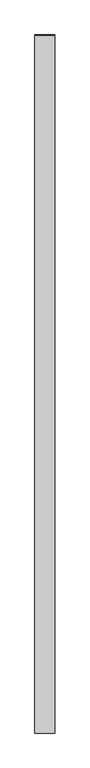
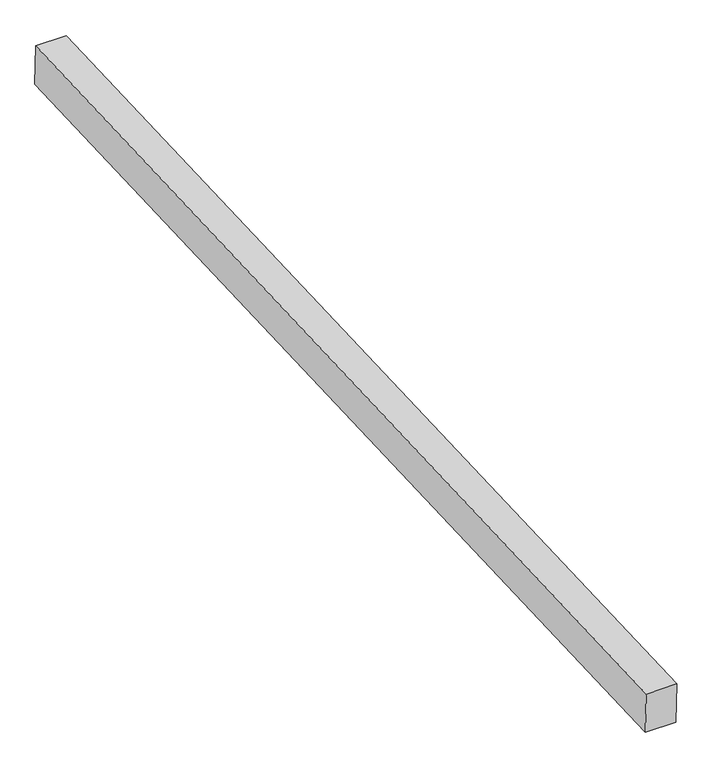
"""IFC4 building model written with IfcOpenShell, lengths in millimetres: proxy geometry, Generic Models 7:Generic Models 1:8:Generic Models 1:8 : Generic Models 7:Generic Models 1:337419:6 : Generic Models 7:Generic Models 1:8:Generic Models 1:8 : Generic Models 7:Generic Models 1:337419:315935."""

from ifc_helpers import new_model, si_unit, frame, origin, place, context, project, spatial, polyline, outline, extrude, source, transform, mapped, element, save


def generic_models_e63649a8(model_context):
    return source(origin(), model_context, "Body", "SweptSolid", [
        extrude(outline(polyline([(-580626.555738, 3844.0209448), (-575753.6328438, 4047.0593987), (-575746.0659221, 3856.7093942), (-580618.6251193, 3653.6860944), (-580626.555738, 3844.0209448)])), frame((593665.061724, 0.0, 0.0), z_axis=(1.0, 0.0, 0.0), x_axis=(0.0, 1.0, 0.0)), (0.0, 0.0, 1.0), 139.7),
    ])


if __name__ == "__main__":
    model = new_model("IFC4")
    model_context = context("Model", 3, world=origin())
    ifc_project = project(units=[si_unit("LENGTHUNIT", "METRE", prefix="MILLI")], contexts=[model_context])
    site = spatial("IfcSite", under=ifc_project)
    building = spatial("IfcBuilding", under=site)
    placement = place(None, origin())
    generic_models_shape = generic_models_e63649a8(model_context)
    element("IfcBuildingElementProxy", 1, Name="Generic Models 7:Generic Models 1:8:Generic Models 1:8 : Generic Models 7:Generic Models 1:337419:6 : Generic Models 7:Generic Models 1:8:Generic Models 1:8 : Generic Models 7:Generic Models 1:337419:315935", ObjectType="Generic Models 7:Generic Models 1:8:Generic Models 1:8 : Generic Models 7:Generic Models 1:337419:6 : Generic Models 7:Generic Models 1:8:Generic Models 1:8 : Generic Models 7:Generic Models 1:337419:315935", at=placement, inside=building, context=model_context, shape_type="MappedRepresentation", body=[
        mapped(generic_models_shape, transform((0.0, 0.0, 0.0), x_axis=(1.0, 0.0, 0.0), y_axis=(0.0, 1.0, 0.0), z_axis=(0.0, 0.0, 1.0))),
    ])
    save(model, "model.ifc")

# Revit data of these elements
# Type "Generic Models 7:Generic Models 1:8:Generic Models 1:8 : Generic Models 7:Generic Models 1:337419:6 : Generic Models 7:Generic Models 1:8:Generic Models 1:8 : Generic Models 7:Generic Models 1:337419:315935"
#   NameOverride = "Generic Models 7:Generic Models 1:8:Generic Models 1:8 : Generic Models 7:Generic Models 1:337419:315935"
#   ObjectTypeOverride = "Generic Models 1:8 : Generic Models 7:Generic Models 1:337419"
#   Reference = "Generic Models 1"
#   Tag = "315935"
# Element 1 (IfcBuildingElementProxy, "Generic Models 7:Generic Models 1:8:Generic Models 1:8 : Generic Models 7:Generic Models 1:337419:6 : Generic Models 7:Generic Models 1:8:Generic Models 1:8 : Generic Models 7:Generic Models 1:337419:315935")
#   Materials on its faces: "5 1/2\" X 7 1/2\" EXTERIOR GRADE GLULAM BEAMS"
# Materials
#   "5 1/2\" X 7 1/2\" EXTERIOR GRADE GLULAM BEAMS": class "Wood", colour RGB 183 134 68, transparency 0, Keynote = "M06181300.01", Description = "Pinus Echinata", Cost = 0
